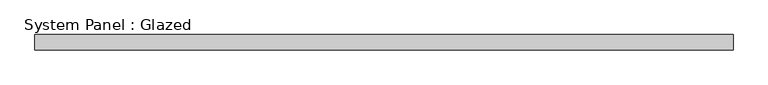
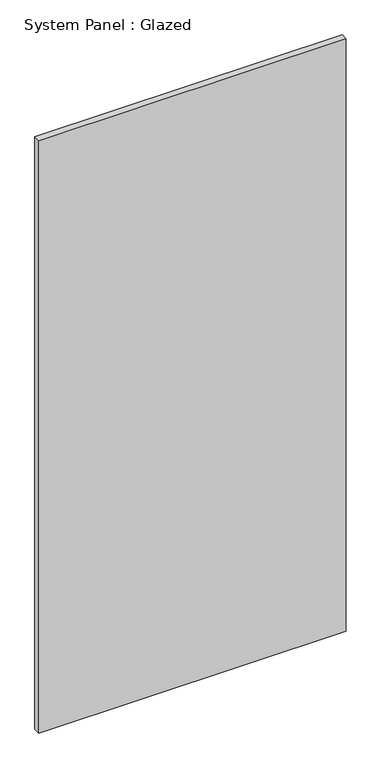
"""IFC4 building model written with IfcOpenShell, lengths in millimetres: plate geometry, System Panel : Glazed."""

import ifcopenshell
import ifcopenshell.guid

model = None  # the IFC model being written
_history = None  # IfcOwnerHistory: only IFC2X3 demands one
_inside = {}  # id of a spatial element -> (the spatial element, [elements in it])
_under = {}  # id of a project, library or spatial element -> (it, [spatial elements below it])
_declared = {}  # id of a project -> (the project, [libraries it declares])
_typed = {}  # id of a type object -> (the type object, [elements of that type])
_made_of = {}  # id of a material, layer set ... -> (it, [elements and type objects made of it])


def new_model(schema):
    """Start an empty IFC model of exactly this schema.

    Asked for "IFC4X3", IfcOpenShell would pick the latest addendum, in which some entities
    have other attributes; the version numbers below select the first issue.
    IFC2X3 requires an IfcOwnerHistory on every rooted entity: one is made here for all.
    """
    global model, _history
    if schema == "IFC4X3":
        model = ifcopenshell.file(schema_version=(4, 3, 0, 0))
    else:
        model = ifcopenshell.file(schema=schema)
    _inside.clear()
    _under.clear()
    _declared.clear()
    _typed.clear()
    _made_of.clear()
    _history = None
    if model.schema == "IFC2X3":
        org = make("IfcOrganization", Name="unknown")
        user = make(
            "IfcPersonAndOrganization",
            ThePerson=make("IfcPerson", FamilyName="unknown"),
            TheOrganization=org,
        )
        app = make(
            "IfcApplication",
            ApplicationDeveloper=org,
            Version="unknown",
            ApplicationFullName="unknown",
            ApplicationIdentifier="unknown",
        )
        _history = make(
            "IfcOwnerHistory",
            OwningUser=user,
            OwningApplication=app,
            ChangeAction="ADDED",
            CreationDate=0,
        )
    return model


def make(cls, **values):
    """One entity of the class cls with the attributes given. An attribute that is None is left unset."""
    return model.create_entity(
        cls, **{name: value for name, value in values.items() if value is not None}
    )


def rooted(cls, **values):
    """An entity with a GlobalId (a new one), such as an element, a storey or a relation."""
    return make(cls, GlobalId=ifcopenshell.guid.new(), OwnerHistory=_history, **values)


def si_unit(unit_type, name, prefix=None):
    """IfcSIUnit, for example si_unit("LENGTHUNIT", "METRE", prefix="MILLI")."""
    return make("IfcSIUnit", UnitType=unit_type, Prefix=prefix, Name=name)


def assignment(units):
    """IfcUnitAssignment: the units of a project."""
    return None if units is None else make("IfcUnitAssignment", Units=units)


def point(xyz):
    """IfcCartesianPoint."""
    return None if xyz is None else make("IfcCartesianPoint", Coordinates=xyz)


def direction(xyz):
    """IfcDirection."""
    return None if xyz is None else make("IfcDirection", DirectionRatios=xyz)


def frame(location, z_axis=None, x_axis=None):
    """IfcAxis2Placement3D, a coordinate frame: its origin and axes. An axis left out is left unset."""
    return make(
        "IfcAxis2Placement3D",
        Location=point(location),
        Axis=direction(z_axis),
        RefDirection=direction(x_axis),
    )


def origin():
    """The frame at (0, 0, 0) with its axes left unset."""
    return frame((0.0, 0.0, 0.0))


def origin_with_axes():
    """The frame at (0, 0, 0) with the z axis (0, 0, 1) and the x axis (1, 0, 0) written out."""
    return frame((0.0, 0.0, 0.0), z_axis=(0.0, 0.0, 1.0), x_axis=(1.0, 0.0, 0.0))


def place(relative_to, where):
    """IfcLocalPlacement: puts the frame where relative to a parent placement (None: the world)."""
    return make(
        "IfcLocalPlacement", PlacementRelTo=relative_to, RelativePlacement=where
    )


def context(
    kind, dimensions, precision=None, world=None, true_north=None, identifier=None
):
    """IfcGeometricRepresentationContext, for example the 3D "Model" context."""
    return make(
        "IfcGeometricRepresentationContext",
        ContextIdentifier=identifier,
        ContextType=kind,
        CoordinateSpaceDimension=dimensions,
        Precision=precision,
        WorldCoordinateSystem=world,
        TrueNorth=true_north,
    )


def project(units=None, contexts=None):
    """IfcProject with its units and contexts."""
    return rooted(
        "IfcProject",
        Name="project",
        RepresentationContexts=contexts,
        UnitsInContext=assignment(units),
    )


def spatial(cls, under=None, at=None, **own):
    """A site, building, storey or space (cls), placed at a placement, below another one or the project."""
    s = rooted(cls, ObjectPlacement=at, **own)
    if under is not None:
        _under.setdefault(under.id(), (under, []))[1].append(s)
    return s


def polyline(points):
    """IfcPolyline through the points."""
    return make("IfcPolyline", Points=[point(p) for p in points])


def outline(outer, holes=None, kind="AREA"):
    """IfcArbitraryClosedProfileDef: a profile drawn as a closed curve; with holes, ...WithVoids."""
    if holes is None:
        return make("IfcArbitraryClosedProfileDef", ProfileType=kind, OuterCurve=outer)
    return make(
        "IfcArbitraryProfileDefWithVoids",
        ProfileType=kind,
        OuterCurve=outer,
        InnerCurves=holes,
    )


def extrude(swept, where, along, depth):
    """IfcExtrudedAreaSolid: the profile swept, set in the frame where, extruded along a direction by depth."""
    return make(
        "IfcExtrudedAreaSolid",
        SweptArea=swept,
        Position=where,
        ExtrudedDirection=direction(along),
        Depth=depth,
    )


def shape(context_of_items, identifier, shape_type, items):
    """IfcShapeRepresentation: the items that make up one representation, for example the "Body"."""
    return make(
        "IfcShapeRepresentation",
        ContextOfItems=context_of_items,
        RepresentationIdentifier=identifier,
        RepresentationType=shape_type,
        Items=items,
    )


def source(mapping_origin, context_of_items, identifier, shape_type, items):
    """IfcRepresentationMap: a shape defined once, which mapped items show again and again."""
    return make(
        "IfcRepresentationMap",
        MappingOrigin=mapping_origin,
        MappedRepresentation=shape(context_of_items, identifier, shape_type, items),
    )


def transform(
    local_origin,
    x_axis=None,
    y_axis=None,
    z_axis=None,
    scale=None,
    scale2=None,
    scale3=None,
    uniform=True,
):
    """IfcCartesianTransformationOperator3D, or its non-uniform kind. x_axis, y_axis, z_axis: its Axis1, 2, 3."""
    if uniform:
        return make(
            "IfcCartesianTransformationOperator3D",
            Axis1=direction(x_axis),
            Axis2=direction(y_axis),
            LocalOrigin=point(local_origin),
            Scale=scale,
            Axis3=direction(z_axis),
        )
    return make(
        "IfcCartesianTransformationOperator3DnonUniform",
        Axis1=direction(x_axis),
        Axis2=direction(y_axis),
        LocalOrigin=point(local_origin),
        Scale=scale,
        Axis3=direction(z_axis),
        Scale2=scale2,
        Scale3=scale3,
    )


def mapped(mapping_source, mapping_target):
    """IfcMappedItem: shows the shape of a source again, moved by a transform."""
    return make(
        "IfcMappedItem", MappingSource=mapping_source, MappingTarget=mapping_target
    )


def made_of(thing, what):
    """Note that an element or type object is made of a material, layer set ...; save() writes the relation."""
    if what is not None:
        _made_of.setdefault(what.id(), (what, []))[1].append(thing)
    return thing


def element(
    cls,
    number,
    at=None,
    inside=None,
    cuts=None,
    type_object=None,
    material=None,
    context=None,
    identifier="Body",
    shape_type=None,
    held_by="IfcProductDefinitionShape",
    body=None,
    shapes=None,
    **own,
):
    """One element of the class cls, such as IfcWall. Its Tag is "e" and its number.

    at: its placement. inside: the storey or other place that contains it. cuts: it is an
    opening in that element (IfcRelVoidsElement). A single representation is given by context,
    identifier, shape_type and body (its items); several are given by shapes. held_by: the class
    of the entity that holds the representations. save() writes the other relations.
    """
    e = rooted(cls, Tag="e%d" % number, ObjectPlacement=at, **own)
    if body is not None:
        shapes = [shape(context, identifier, shape_type, body)]
    if shapes is not None:
        e.Representation = make(held_by, Representations=shapes)
    if inside is not None:
        _inside.setdefault(inside.id(), (inside, []))[1].append(e)
    if cuts is not None:
        rooted(
            "IfcRelVoidsElement", RelatingBuildingElement=cuts, RelatedOpeningElement=e
        )
    if type_object is not None:
        _typed.setdefault(type_object.id(), (type_object, []))[1].append(e)
    return made_of(e, material)


def aggregate(whole, parts):
    """IfcRelAggregates: a whole, such as a stair, and the parts it consists of."""
    return rooted("IfcRelAggregates", RelatingObject=whole, RelatedObjects=parts)


def save(model, path):
    """Write the relations noted so far, then the file.

    IfcRelAggregates (storeys below a building ...), IfcRelContainedInSpatialStructure (elements
    in a storey), IfcRelDefinesByType, IfcRelAssociatesMaterial and IfcRelDeclares: one each for
    every whole, place, type object, material and project.
    """
    for whole, parts in _under.values():
        aggregate(whole, parts)
    for where, things in _inside.values():
        rooted(
            "IfcRelContainedInSpatialStructure",
            RelatedElements=things,
            RelatingStructure=where,
        )
    for kind, things in _typed.values():
        rooted("IfcRelDefinesByType", RelatedObjects=things, RelatingType=kind)
    for what, things in _made_of.values():
        rooted("IfcRelAssociatesMaterial", RelatedObjects=things, RelatingMaterial=what)
    for by, libraries in _declared.values():
        rooted("IfcRelDeclares", RelatingContext=by, RelatedDefinitions=libraries)
    model.write(path)


def system_panel_glazed_f2541063(model_context):
    return source(origin(), model_context, "Body", "SweptSolid", [
        extrude(outline(polyline([(583.1416667, 19.05), (-583.1416667, 19.05), (-583.1416667, 44.45), (583.1416667, 44.45), (583.1416667, 19.05)])), origin_with_axes(), (0.0, 0.0, 1.0), 2374.9),
    ])


if __name__ == "__main__":
    model = new_model("IFC4")
    model_context = context("Model", 3, world=origin())
    ifc_project = project(units=[si_unit("LENGTHUNIT", "METRE", prefix="MILLI")], contexts=[model_context])
    site = spatial("IfcSite", under=ifc_project)
    building = spatial("IfcBuilding", under=site)
    placement = place(None, origin())
    system_panel_glazed_shape = system_panel_glazed_f2541063(model_context)
    element("IfcPlate", 1, ObjectType="System Panel : Glazed", at=placement, inside=building, context=model_context, shape_type="MappedRepresentation", body=[
        mapped(system_panel_glazed_shape, transform((0.0, 0.0, 0.0), x_axis=(1.0, 0.0, 0.0), y_axis=(0.0, 1.0, 0.0), z_axis=(0.0, 0.0, 1.0))),
    ])
    save(model, "model.ifc")

# Revit data of these elements
# Element 1 (IfcPlate, "System Panel : Glazed")
#   Materials on its faces: "Glass"
# Materials
#   "Glass": class "Glass", colour RGB 218 227 224, transparency 0.85, Description = "Soda Lime Glass", Cost = 0
